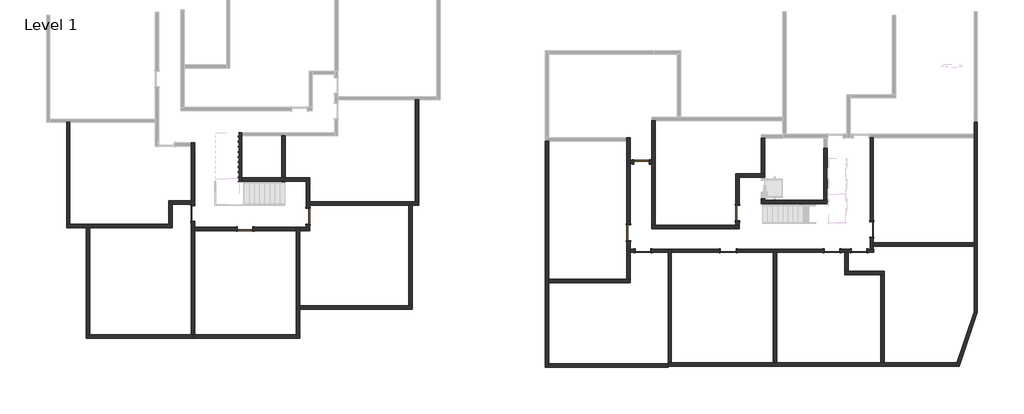
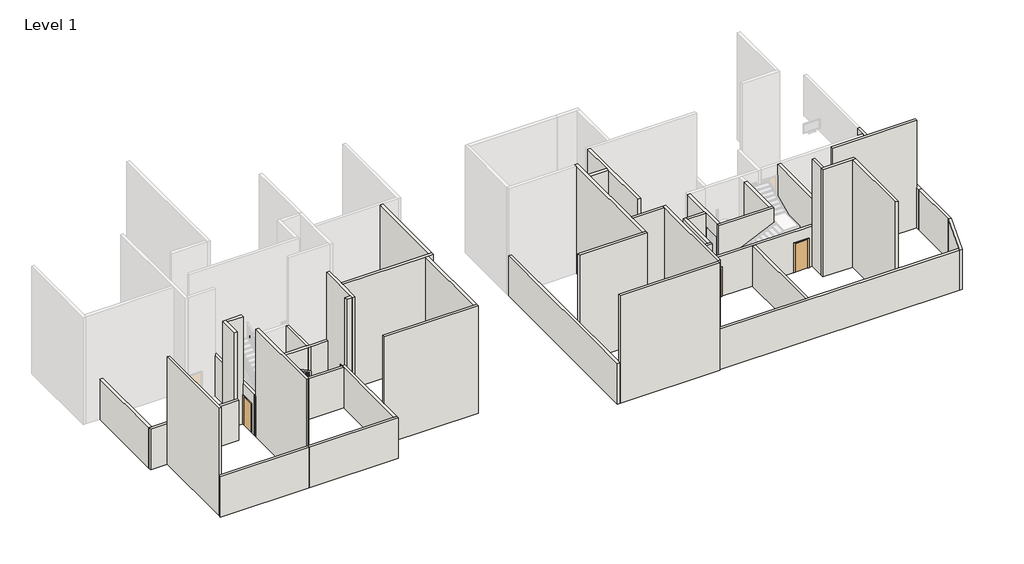
# One storey, part 1 of 3: 45 walls, 11 doors.
"""IFC4 building model written with IfcOpenShell, lengths in millimetres."""

import ifcopenshell
import ifcopenshell.guid

model = None  # the IFC model being written
_history = None  # IfcOwnerHistory: only IFC2X3 demands one
_inside = {}  # id of a spatial element -> (the spatial element, [elements in it])
_under = {}  # id of a project, library or spatial element -> (it, [spatial elements below it])
_declared = {}  # id of a project -> (the project, [libraries it declares])
_typed = {}  # id of a type object -> (the type object, [elements of that type])
_made_of = {}  # id of a material, layer set ... -> (it, [elements and type objects made of it])


def new_model(schema):
    """Start an empty IFC model of exactly this schema.

    Asked for "IFC4X3", IfcOpenShell would pick the latest addendum, in which some entities
    have other attributes; the version numbers below select the first issue.
    IFC2X3 requires an IfcOwnerHistory on every rooted entity: one is made here for all.
    """
    global model, _history
    if schema == "IFC4X3":
        model = ifcopenshell.file(schema_version=(4, 3, 0, 0))
    else:
        model = ifcopenshell.file(schema=schema)
    _inside.clear()
    _under.clear()
    _declared.clear()
    _typed.clear()
    _made_of.clear()
    _history = None
    if model.schema == "IFC2X3":
        org = make("IfcOrganization", Name="unknown")
        user = make(
            "IfcPersonAndOrganization",
            ThePerson=make("IfcPerson", FamilyName="unknown"),
            TheOrganization=org,
        )
        app = make(
            "IfcApplication",
            ApplicationDeveloper=org,
            Version="unknown",
            ApplicationFullName="unknown",
            ApplicationIdentifier="unknown",
        )
        _history = make(
            "IfcOwnerHistory",
            OwningUser=user,
            OwningApplication=app,
            ChangeAction="ADDED",
            CreationDate=0,
        )
    return model


def make(cls, **values):
    """One entity of the class cls with the attributes given. An attribute that is None is left unset."""
    return model.create_entity(
        cls, **{name: value for name, value in values.items() if value is not None}
    )


def rooted(cls, **values):
    """An entity with a GlobalId (a new one), such as an element, a storey or a relation."""
    return make(cls, GlobalId=ifcopenshell.guid.new(), OwnerHistory=_history, **values)


def si_unit(unit_type, name, prefix=None):
    """IfcSIUnit, for example si_unit("LENGTHUNIT", "METRE", prefix="MILLI")."""
    return make("IfcSIUnit", UnitType=unit_type, Prefix=prefix, Name=name)


def assignment(units):
    """IfcUnitAssignment: the units of a project."""
    return None if units is None else make("IfcUnitAssignment", Units=units)


def point(xyz):
    """IfcCartesianPoint."""
    return None if xyz is None else make("IfcCartesianPoint", Coordinates=xyz)


def direction(xyz):
    """IfcDirection."""
    return None if xyz is None else make("IfcDirection", DirectionRatios=xyz)


def frame(location, z_axis=None, x_axis=None):
    """IfcAxis2Placement3D, a coordinate frame: its origin and axes. An axis left out is left unset."""
    return make(
        "IfcAxis2Placement3D",
        Location=point(location),
        Axis=direction(z_axis),
        RefDirection=direction(x_axis),
    )


def origin():
    """The frame at (0, 0, 0) with its axes left unset."""
    return frame((0.0, 0.0, 0.0))


def origin_with_axes():
    """The frame at (0, 0, 0) with the z axis (0, 0, 1) and the x axis (1, 0, 0) written out."""
    return frame((0.0, 0.0, 0.0), z_axis=(0.0, 0.0, 1.0), x_axis=(1.0, 0.0, 0.0))


def place(relative_to, where):
    """IfcLocalPlacement: puts the frame where relative to a parent placement (None: the world)."""
    return make(
        "IfcLocalPlacement", PlacementRelTo=relative_to, RelativePlacement=where
    )


def context(
    kind, dimensions, precision=None, world=None, true_north=None, identifier=None
):
    """IfcGeometricRepresentationContext, for example the 3D "Model" context."""
    return make(
        "IfcGeometricRepresentationContext",
        ContextIdentifier=identifier,
        ContextType=kind,
        CoordinateSpaceDimension=dimensions,
        Precision=precision,
        WorldCoordinateSystem=world,
        TrueNorth=true_north,
    )


def project(units=None, contexts=None):
    """IfcProject with its units and contexts."""
    return rooted(
        "IfcProject",
        Name="project",
        RepresentationContexts=contexts,
        UnitsInContext=assignment(units),
    )


def spatial(cls, under=None, at=None, **own):
    """A site, building, storey or space (cls), placed at a placement, below another one or the project."""
    s = rooted(cls, ObjectPlacement=at, **own)
    if under is not None:
        _under.setdefault(under.id(), (under, []))[1].append(s)
    return s


def polyline(points):
    """IfcPolyline through the points."""
    return make("IfcPolyline", Points=[point(p) for p in points])


def outline(outer, holes=None, kind="AREA"):
    """IfcArbitraryClosedProfileDef: a profile drawn as a closed curve; with holes, ...WithVoids."""
    if holes is None:
        return make("IfcArbitraryClosedProfileDef", ProfileType=kind, OuterCurve=outer)
    return make(
        "IfcArbitraryProfileDefWithVoids",
        ProfileType=kind,
        OuterCurve=outer,
        InnerCurves=holes,
    )


def extrude(swept, where, along, depth):
    """IfcExtrudedAreaSolid: the profile swept, set in the frame where, extruded along a direction by depth."""
    return make(
        "IfcExtrudedAreaSolid",
        SweptArea=swept,
        Position=where,
        ExtrudedDirection=direction(along),
        Depth=depth,
    )


def faces_of(points, faces, orient=None, outer=None):
    """IfcFace entities. A face is a list of loops; a loop is a list of indices into points, from 0.

    orient and outer hold one flag for each loop. By default every Orientation is true, the
    first loop of a face is its IfcFaceOuterBound and the others are IfcFaceBound.
    """
    made = []
    for i, loops in enumerate(faces):
        bounds = []
        for j, loop in enumerate(loops):
            is_outer = j == 0 if outer is None else outer[i][j]
            bounds.append(
                make(
                    "IfcFaceOuterBound" if is_outer else "IfcFaceBound",
                    Bound=make("IfcPolyLoop", Polygon=[points[k] for k in loop]),
                    Orientation=True if orient is None else orient[i][j],
                )
            )
        made.append(make("IfcFace", Bounds=bounds))
    return made


def faceted_brep(points, faces, orient=None, outer=None, voids=None):
    """IfcFacetedBrep: a solid bounded by flat faces; with voids (closed shells), ...WithVoids."""
    shared = [point(p) for p in points]
    hull = make("IfcClosedShell", CfsFaces=faces_of(shared, faces, orient, outer))
    if voids is None:
        return make("IfcFacetedBrep", Outer=hull)
    return make(
        "IfcFacetedBrepWithVoids",
        Outer=hull,
        Voids=[
            make(cls, CfsFaces=faces_of(shared, fs, o, b)) for cls, fs, o, b in voids
        ],
    )


def shape(context_of_items, identifier, shape_type, items):
    """IfcShapeRepresentation: the items that make up one representation, for example the "Body"."""
    return make(
        "IfcShapeRepresentation",
        ContextOfItems=context_of_items,
        RepresentationIdentifier=identifier,
        RepresentationType=shape_type,
        Items=items,
    )


def source(mapping_origin, context_of_items, identifier, shape_type, items):
    """IfcRepresentationMap: a shape defined once, which mapped items show again and again."""
    return make(
        "IfcRepresentationMap",
        MappingOrigin=mapping_origin,
        MappedRepresentation=shape(context_of_items, identifier, shape_type, items),
    )


def transform(
    local_origin,
    x_axis=None,
    y_axis=None,
    z_axis=None,
    scale=None,
    scale2=None,
    scale3=None,
    uniform=True,
):
    """IfcCartesianTransformationOperator3D, or its non-uniform kind. x_axis, y_axis, z_axis: its Axis1, 2, 3."""
    if uniform:
        return make(
            "IfcCartesianTransformationOperator3D",
            Axis1=direction(x_axis),
            Axis2=direction(y_axis),
            LocalOrigin=point(local_origin),
            Scale=scale,
            Axis3=direction(z_axis),
        )
    return make(
        "IfcCartesianTransformationOperator3DnonUniform",
        Axis1=direction(x_axis),
        Axis2=direction(y_axis),
        LocalOrigin=point(local_origin),
        Scale=scale,
        Axis3=direction(z_axis),
        Scale2=scale2,
        Scale3=scale3,
    )


def mapped(mapping_source, mapping_target):
    """IfcMappedItem: shows the shape of a source again, moved by a transform."""
    return make(
        "IfcMappedItem", MappingSource=mapping_source, MappingTarget=mapping_target
    )


def made_of(thing, what):
    """Note that an element or type object is made of a material, layer set ...; save() writes the relation."""
    if what is not None:
        _made_of.setdefault(what.id(), (what, []))[1].append(thing)
    return thing


def element(
    cls,
    number,
    at=None,
    inside=None,
    cuts=None,
    type_object=None,
    material=None,
    context=None,
    identifier="Body",
    shape_type=None,
    held_by="IfcProductDefinitionShape",
    body=None,
    shapes=None,
    **own,
):
    """One element of the class cls, such as IfcWall. Its Tag is "e" and its number.

    at: its placement. inside: the storey or other place that contains it. cuts: it is an
    opening in that element (IfcRelVoidsElement). A single representation is given by context,
    identifier, shape_type and body (its items); several are given by shapes. held_by: the class
    of the entity that holds the representations. save() writes the other relations.
    """
    e = rooted(cls, Tag="e%d" % number, ObjectPlacement=at, **own)
    if body is not None:
        shapes = [shape(context, identifier, shape_type, body)]
    if shapes is not None:
        e.Representation = make(held_by, Representations=shapes)
    if inside is not None:
        _inside.setdefault(inside.id(), (inside, []))[1].append(e)
    if cuts is not None:
        rooted(
            "IfcRelVoidsElement", RelatingBuildingElement=cuts, RelatedOpeningElement=e
        )
    if type_object is not None:
        _typed.setdefault(type_object.id(), (type_object, []))[1].append(e)
    return made_of(e, material)


def aggregate(whole, parts):
    """IfcRelAggregates: a whole, such as a stair, and the parts it consists of."""
    return rooted("IfcRelAggregates", RelatingObject=whole, RelatedObjects=parts)


def save(model, path):
    """Write the relations noted so far, then the file.

    IfcRelAggregates (storeys below a building ...), IfcRelContainedInSpatialStructure (elements
    in a storey), IfcRelDefinesByType, IfcRelAssociatesMaterial and IfcRelDeclares: one each for
    every whole, place, type object, material and project.
    """
    for whole, parts in _under.values():
        aggregate(whole, parts)
    for where, things in _inside.values():
        rooted(
            "IfcRelContainedInSpatialStructure",
            RelatedElements=things,
            RelatingStructure=where,
        )
    for kind, things in _typed.values():
        rooted("IfcRelDefinesByType", RelatedObjects=things, RelatingType=kind)
    for what, things in _made_of.values():
        rooted("IfcRelAssociatesMaterial", RelatedObjects=things, RelatingMaterial=what)
    for by, libraries in _declared.values():
        rooted("IfcRelDeclares", RelatingContext=by, RelatedDefinitions=libraries)
    model.write(path)


def m_single_flush_0915_x_2134mm_727434cd(model_context):
    return source(origin(), model_context, "Body", "SweptSolid", [
        extrude(outline(polyline([(2210.0, -533.5), (0.0, -533.5), (0.0, -457.5), (2134.0, -457.5), (2134.0, 457.5), (0.0, 457.5), (0.0, 533.5), (2210.0, 533.5), (2210.0, -533.5)])), frame((0.0, -125.0, 0.0), z_axis=(0.0, 1.0, 0.0), x_axis=(0.0, 0.0, 1.0)), (0.0, 0.0, 1.0), 25.0),
        extrude(outline(polyline([(2210.0, 533.5), (2210.0, -533.5), (0.0, -533.5), (0.0, -457.5), (2134.0, -457.5), (2134.0, 457.5), (0.0, 457.5), (0.0, 533.5), (2210.0, 533.5)])), frame((0.0, 100.0, 0.0), z_axis=(0.0, 1.0, 0.0), x_axis=(0.0, 0.0, 1.0)), (0.0, 0.0, 1.0), 25.0),
        extrude(outline(polyline([(457.5, -49.0), (457.5, -100.0), (-457.5, -100.0), (-457.5, -49.0), (457.5, -49.0)])), origin_with_axes(), (0.0, 0.0, 1.0), 2134.0),
    ])


def m_single_flush_0915_x_2134mm_6a9e8738(model_context):
    return source(origin(), model_context, "Body", "SweptSolid", [
        extrude(outline(polyline([(2210.0, -533.5), (0.0, -533.5), (0.0, -457.5), (2134.0, -457.5), (2134.0, 457.5), (0.0, 457.5), (0.0, 533.5), (2210.0, 533.5), (2210.0, -533.5)])), frame((0.0, 100.0, 0.0), z_axis=(0.0, 1.0, 0.0), x_axis=(0.0, 0.0, 1.0)), (0.0, 0.0, 1.0), 25.0),
        extrude(outline(polyline([(2210.0, 533.5), (2210.0, -533.5), (0.0, -533.5), (0.0, -457.5), (2134.0, -457.5), (2134.0, 457.5), (0.0, 457.5), (0.0, 533.5), (2210.0, 533.5)])), frame((0.0, -125.0, 0.0), z_axis=(0.0, 1.0, 0.0), x_axis=(0.0, 0.0, 1.0)), (0.0, 0.0, 1.0), 25.0),
        extrude(outline(polyline([(457.5, 49.0), (-457.5, 49.0), (-457.5, 100.0), (457.5, 100.0), (457.5, 49.0)])), origin_with_axes(), (0.0, 0.0, 1.0), 2134.0),
    ])


model = new_model("IFC4")

# Units and contexts
model_context = context("Model", 3, world=origin())
ifc_project = project(units=[si_unit("LENGTHUNIT", "METRE", prefix="MILLI")], contexts=[model_context])

# Site, building, storey
site = spatial("IfcSite", under=ifc_project)
building = spatial("IfcBuilding", under=site)
storey = spatial("IfcBuildingStorey", under=building, Name="Level 1", Elevation=0.0)

# Doors
placement = place(None, origin())
m_single_flush_0915_x_2134mm_shape = m_single_flush_0915_x_2134mm_727434cd(model_context)
element("IfcDoor", 1, ObjectType="M_Single-Flush : 0915 x 2134mm", at=placement, inside=storey, context=model_context, shape_type="MappedRepresentation", body=[
    mapped(m_single_flush_0915_x_2134mm_shape, transform((16150.6041014, -4023.024372, 0.0), x_axis=(0.0, -1.0, 0.0), y_axis=(1.0, 0.0, 0.0), z_axis=(0.0, 0.0, 1.0))),
])
element("IfcDoor", 2, ObjectType="M_Single-Flush : 0915 x 2134mm", at=placement, inside=storey, context=model_context, shape_type="MappedRepresentation", body=[
    mapped(m_single_flush_0915_x_2134mm_shape, transform((15602.336337, -6240.0098119, 0.0), x_axis=(1.0, 0.0, 0.0), y_axis=(0.0, 1.0, 0.0), z_axis=(0.0, 0.0, 1.0))),
])
element("IfcDoor", 3, ObjectType="M_Single-Flush : 0915 x 2134mm", at=placement, inside=storey, context=model_context, shape_type="MappedRepresentation", body=[
    mapped(m_single_flush_0915_x_2134mm_shape, transform((21711.3612349, -6240.0098119, 0.0), x_axis=(1.0, 0.0, 0.0), y_axis=(0.0, 1.0, 0.0), z_axis=(0.0, 0.0, 1.0))),
])
element("IfcDoor", 4, ObjectType="M_Single-Flush : 0915 x 2134mm", at=placement, inside=storey, context=model_context, shape_type="MappedRepresentation", body=[
    mapped(m_single_flush_0915_x_2134mm_shape, transform((-9130.3629108, -4209.1627129, 0.0), x_axis=(0.0, 1.0, 0.0), y_axis=(-1.0, 0.0, 0.0), z_axis=(0.0, 0.0, 1.0))),
])
m_single_flush_0915_x_2134mm_2_shape = m_single_flush_0915_x_2134mm_6a9e8738(model_context)
element("IfcDoor", 5, ObjectType="M_Single-Flush : 0915 x 2134mm", at=placement, inside=storey, context=model_context, shape_type="MappedRepresentation", body=[
    mapped(m_single_flush_0915_x_2134mm_2_shape, transform((24048.8612349, -4982.5098119, 0.0), x_axis=(0.0, -1.0, 0.0), y_axis=(1.0, 0.0, 0.0), z_axis=(0.0, 0.0, 1.0))),
])
element("IfcDoor", 6, ObjectType="M_Single-Flush : 0915 x 2134mm", at=placement, inside=storey, context=model_context, shape_type="MappedRepresentation", body=[
    mapped(m_single_flush_0915_x_2134mm_2_shape, transform((23308.8612349, -6240.0098119, 0.0), x_axis=(-1.0, 0.0, 0.0), y_axis=(0.0, -1.0, 0.0), z_axis=(0.0, 0.0, 1.0))),
])
element("IfcDoor", 7, ObjectType="M_Single-Flush : 0915 x 2134mm", at=placement, inside=storey, context=model_context, shape_type="MappedRepresentation", body=[
    mapped(m_single_flush_0915_x_2134mm_2_shape, transform((-12832.3304233, -4959.1627129, 0.0), x_axis=(-1.0, 0.0, 0.0), y_axis=(0.0, -1.0, 0.0), z_axis=(0.0, 0.0, 1.0))),
])
element("IfcDoor", 8, ObjectType="M_Single-Flush : 0915 x 2134mm", at=placement, inside=storey, context=model_context, shape_type="MappedRepresentation", body=[
    mapped(m_single_flush_0915_x_2134mm_2_shape, transform((10586.3612349, -6236.6907835, 0.0), x_axis=(-1.0, 0.0, 0.0), y_axis=(0.0, -1.0, 0.0), z_axis=(0.0, 0.0, 1.0))),
])
element("IfcDoor", 9, ObjectType="M_Single-Flush : 0915 x 2134mm", at=placement, inside=storey, context=model_context, shape_type="MappedRepresentation", body=[
    mapped(m_single_flush_0915_x_2134mm_2_shape, transform((9728.8612349, -5179.1907835, 0.0), x_axis=(0.0, 1.0, 0.0), y_axis=(-1.0, 0.0, 0.0), z_axis=(0.0, 0.0, 1.0))),
])
element("IfcDoor", 10, ObjectType="M_Single-Flush : 0915 x 2134mm", at=placement, inside=storey, context=model_context, shape_type="MappedRepresentation", body=[
    mapped(m_single_flush_0915_x_2134mm_2_shape, transform((10497.5506524, -1020.524372, 0.0), x_axis=(1.0, 0.0, 0.0), y_axis=(0.0, 1.0, 0.0), z_axis=(0.0, 0.0, 1.0))),
])
element("IfcDoor", 11, ObjectType="M_Single-Flush : 0915 x 2134mm", at=placement, inside=storey, context=model_context, shape_type="MappedRepresentation", body=[
    mapped(m_single_flush_0915_x_2134mm_2_shape, transform((-15913.9741722, -4044.6599715, 0.0), x_axis=(0.0, 1.0, 0.0), y_axis=(-1.0, 0.0, 0.0), z_axis=(0.0, 0.0, 1.0))),
])

# Walls
element("IfcWall", 12, ObjectType="Generic - 200mm", at=placement, inside=storey, context=model_context, shape_type="Brep", body=[
    faceted_brep([(30068.8612349, 1319.475628, 0.0), (30068.8612349, 619.475628, 0.0), (30068.8612349, 419.475628, 0.0), (30068.8612349, -5760.0098119, 0.0), (30068.8612349, -5960.0098119, 0.0), (30068.8612349, -6240.0098119, 0.0), (30068.8612349, -6240.0098119, 3000.0), (30068.8612349, 419.475628, 3000.0), (30068.8612349, 619.475628, 3000.0), (30068.8612349, 1319.475628, 3000.0), (30268.8612349, 1319.475628, 0.0), (30268.8612349, 1319.475628, 3000.0), (30268.8612349, -6240.0098119, 3000.0), (30268.8612349, -6240.0098119, 0.0), (30268.3425199, 1319.475628, 0.0), (30069.3799498, -6240.0098119, 0.0), (30069.3799498, -6240.0098119, 3000.0), (30268.3425199, 1319.475628, 3000.0)], [[[0, 1, 2, 3, 4, 5, 6, 7, 8, 9]], [[10, 11, 12, 13]], [[5, 4, 3, 2, 1, 0, 14, 10, 13, 15]], [[6, 5, 15, 13, 12, 16]], [[9, 8, 7, 6, 16, 12, 11, 17]], [[0, 9, 17, 11, 10, 14]]]),
])
element("IfcWall", 13, ObjectType="Generic - 200mm", at=placement, inside=storey, context=model_context, shape_type="Brep", body=[
    faceted_brep([(30069.3799498, -6240.0098119, 0.0), (30069.3799498, -9831.8731192, 0.0), (30069.3799498, -9831.8731192, 3000.0), (30069.3799498, -6240.0098119, 3000.0), (30269.3799498, -6240.0098119, 0.0), (30269.3799498, -6240.0098119, 3000.0), (30269.3799498, -9864.7113693, 3000.0), (30269.3799498, -9864.7113693, 0.0), (30268.8612349, -6240.0098119, 0.0), (30268.8612349, -6240.0098119, 3000.0)], [[[0, 1, 2, 3]], [[4, 5, 6, 7]], [[1, 0, 8, 4, 7]], [[3, 2, 6, 5, 9]], [[0, 3, 9, 5, 4, 8]], [[2, 1, 7, 6]]]),
])
element("IfcWall", 14, ObjectType="Generic - 200mm", at=placement, inside=storey, context=model_context, shape_type="Brep", body=[
    faceted_brep([(21429.836337, -3276.2808257, 0.0), (21229.836337, -3276.2808257, 0.0), (17750.6041014, -3276.2808257, 0.0), (17550.6041014, -3276.2808257, 0.0), (17550.6041014, -3276.2808257, 3000.0), (17750.6041014, -3276.2808257, 3000.0), (21229.836337, -3276.2808257, 3000.0), (21429.836337, -3276.2808257, 3000.0), (21429.836337, -3476.2808257, 0.0), (21429.836337, -3476.2808257, 3000.0), (17550.6041014, -3476.2808257, 3000.0), (17550.6041014, -3476.2808257, 0.0)], [[[0, 1, 2, 3, 4, 5, 6, 7]], [[8, 9, 10, 11]], [[3, 2, 1, 0, 8, 11]], [[7, 6, 5, 4, 10, 9]], [[0, 7, 9, 8]], [[4, 3, 11, 10]]]),
])
element("IfcWall", 15, ObjectType="Generic - 200mm", at=placement, inside=storey, context=model_context, shape_type="SweptSolid", body=[
    extrude(outline(polyline([(18459.836337, -6340.0098119), (18459.836337, -12836.6907835), (18259.836337, -12836.6907835), (18259.836337, -6340.0098119), (18459.836337, -6340.0098119)])), origin_with_axes(), (0.0, 0.0, 1.0), 3000.0),
])
element("IfcWall", 16, ObjectType="Generic - 200mm", at=placement, inside=storey, context=model_context, shape_type="Brep", body=[
    faceted_brep([(29055.3124022, -12836.6907835, 0.0), (24788.8612349, -12836.6907835, 0.0), (24588.8612349, -12836.6907835, 0.0), (18459.836337, -12836.6907835, 0.0), (18259.836337, -12836.6907835, 0.0), (12259.836337, -12836.6907835, 0.0), (12059.836337, -12836.6907835, 0.0), (12059.836337, -12836.6907835, 3000.0), (18259.836337, -12836.6907835, 3000.0), (18459.836337, -12836.6907835, 3000.0), (29055.3124022, -12836.6907835, 3000.0), (28987.8162902, -13036.6907835, 0.0), (28987.8162902, -13036.6907835, 3000.0), (12059.836337, -13036.6907835, 3000.0), (12059.836337, -13036.6907835, 0.0), (12059.836337, -12889.1627129, 0.0)], [[[0, 1, 2, 3, 4, 5, 6, 7, 8, 9, 10]], [[11, 12, 13, 14]], [[6, 5, 4, 3, 2, 1, 0, 11, 14, 15]], [[10, 9, 8, 7, 13, 12]], [[0, 10, 12, 11]], [[7, 6, 15, 14, 13]]]),
])
element("IfcWall", 17, ObjectType="Generic - 200mm", at=placement, inside=storey, context=model_context, shape_type="Brep", body=[
    faceted_brep([(30069.3799498, -9831.8731192, 0.0), (29055.3124022, -12836.6907835, 0.0), (28987.8162902, -13036.6907835, 0.0), (28987.8162902, -13036.6907835, 3000.0), (29055.3124022, -12836.6907835, 3000.0), (30069.3799498, -9831.8731192, 3000.0), (30269.3799498, -9864.7113693, 0.0), (30269.3799498, -9864.7113693, 3000.0), (29198.8985612, -13036.6907835, 3000.0), (29198.8985612, -13036.6907835, 0.0)], [[[0, 1, 2, 3, 4, 5]], [[6, 7, 8, 9]], [[2, 1, 0, 6, 9]], [[5, 4, 3, 8, 7]], [[0, 5, 7, 6]], [[3, 2, 9, 8]]]),
])
element("IfcWall", 18, ObjectType="Generic - 200mm", at=placement, inside=storey, context=model_context, shape_type="Brep", body=[
    faceted_brep([(22851.3612349, -6140.0098119, 0.0), (22168.8612349, -6140.0098119, 0.0), (22168.8612349, -6140.0098119, 2134.0), (21253.8612349, -6140.0098119, 2134.0), (21253.8612349, -6140.0098119, 0.0), (16059.836337, -6140.0098119, 0.0), (16059.836337, -6140.0098119, 2134.0), (15144.836337, -6140.0098119, 2134.0), (15144.836337, -6140.0098119, 0.0), (12259.836337, -6140.0098119, 0.0), (12259.836337, -6140.0098119, 3000.0), (23948.8612349, -6140.0098119, 3000.0), (24148.8612349, -6140.0098119, 3000.0), (24163.3998354, -6140.0098119, 3000.0), (24163.3998354, -6140.0098119, 0.0), (24148.8612349, -6140.0098119, 0.0), (23948.8612349, -6140.0098119, 0.0), (23766.3612349, -6140.0098119, 0.0), (23766.3612349, -6140.0098119, 2134.0), (22851.3612349, -6140.0098119, 2134.0), (22168.8612349, -6340.0098119, 2134.0), (22168.8612349, -6340.0098119, 0.0), (22468.8612349, -6340.0098119, 0.0), (22668.8612349, -6340.0098119, 0.0), (22851.3612349, -6340.0098119, 0.0), (22851.3612349, -6340.0098119, 2134.0), (23766.3612349, -6340.0098119, 2134.0), (23766.3612349, -6340.0098119, 0.0), (24163.3998354, -6340.0098119, 0.0), (24163.3998354, -6340.0098119, 3000.0), (18459.836337, -6340.0098119, 3000.0), (18259.836337, -6340.0098119, 3000.0), (12259.836337, -6340.0098119, 3000.0), (12259.836337, -6340.0098119, 0.0), (15144.836337, -6340.0098119, 0.0), (15144.836337, -6340.0098119, 2134.0), (16059.836337, -6340.0098119, 2134.0), (16059.836337, -6340.0098119, 0.0), (18259.836337, -6340.0098119, 0.0), (18459.836337, -6340.0098119, 0.0), (21253.8612349, -6340.0098119, 0.0), (21253.8612349, -6340.0098119, 2134.0)], [[[0, 1, 2, 3, 4, 5, 6, 7, 8, 9, 10, 11, 12, 13, 14, 15, 16, 17, 18, 19]], [[20, 21, 22, 23, 24, 25, 26, 27, 28, 29, 30, 31, 32, 33, 34, 35, 36, 37, 38, 39, 40, 41]], [[17, 16, 15, 14, 28, 27]], [[33, 9, 8, 34]], [[40, 39, 38, 37, 5, 4]], [[24, 23, 22, 21, 1, 0]], [[13, 12, 11, 10, 32, 31, 30, 29]], [[14, 13, 29, 28]], [[36, 6, 5, 37]], [[7, 35, 34, 8]], [[35, 7, 6, 36]], [[25, 24, 0, 19]], [[26, 25, 19, 18]], [[27, 26, 18, 17]], [[10, 9, 33, 32]], [[2, 1, 21, 20]], [[3, 2, 20, 41]], [[4, 3, 41, 40]]]),
])
element("IfcWall", 19, ObjectType="Generic - 200mm", at=placement, inside=storey, context=model_context, shape_type="Brep", body=[
    faceted_brep([(4843.716007, 199.9901881, 0.0), (4843.716007, -13089.1627129, 0.0), (4843.716007, -13089.1627129, 3000.0), (4843.716007, 199.9901881, 3000.0), (5043.716007, 199.9901881, 0.0), (5043.716007, 199.9901881, 3000.0), (5043.716007, -13089.1627129, 3000.0), (5043.716007, -13089.1627129, 0.0), (5043.716007, -12889.1627129, 0.0), (5043.716007, -8120.0098119, 0.0), (5043.716007, -7920.0098119, 0.0)], [[[0, 1, 2, 3]], [[4, 5, 6, 7, 8, 9, 10]], [[1, 0, 4, 10, 9, 8, 7]], [[3, 2, 6, 5]], [[0, 3, 5, 4]], [[2, 1, 7, 6]]]),
])
element("IfcWall", 20, ObjectType="Generic - 200mm", at=placement, inside=storey, context=model_context, shape_type="Brep", body=[
    faceted_brep([(24148.8612349, 419.475628, 3000.0), (24148.8612349, -6140.0098119, 3000.0), (24148.8612349, -6140.0098119, 0.0), (24148.8612349, -5960.0098119, 0.0), (24148.8612349, -5760.0098119, 0.0), (24148.8612349, -5440.0098119, 0.0), (24148.8612349, -5440.0098119, 2134.0), (24148.8612349, -4525.0098119, 2134.0), (24148.8612349, -4525.0098119, 0.0), (24148.8612349, 419.475628, 0.0), (23948.8612349, -6140.0098119, 3000.0), (23948.8612349, 419.475628, 3000.0), (23948.8612349, 419.475628, 0.0), (23948.8612349, -4525.0098119, 0.0), (23948.8612349, -4525.0098119, 2134.0), (23948.8612349, -5440.0098119, 2134.0), (23948.8612349, -5440.0098119, 0.0), (23948.8612349, -6140.0098119, 0.0)], [[[0, 1, 2, 3, 4, 5, 6, 7, 8, 9]], [[10, 11, 12, 13, 14, 15, 16, 17]], [[12, 9, 8, 13]], [[2, 17, 16, 5, 4, 3]], [[1, 0, 11, 10]], [[0, 9, 12, 11]], [[15, 6, 5, 16]], [[7, 14, 13, 8]], [[14, 7, 6, 15]], [[2, 1, 10, 17]]]),
])
element("IfcWall", 21, ObjectType="Generic - 200mm", at=placement, inside=storey, context=model_context, shape_type="SweptSolid", body=[
    extrude(outline(polyline([(21229.836337, -3276.2808257), (21229.836337, -200.524372), (21429.836337, -200.524372), (21429.836337, -3276.2808257), (21229.836337, -3276.2808257)])), origin_with_axes(), (0.0, 0.0, 1.0), 3000.0),
])
element("IfcWall", 22, ObjectType="Generic - 200mm", at=placement, inside=storey, context=model_context, shape_type="Brep", body=[
    faceted_brep([(17550.6041014, -3276.2808257, 3000.0), (17550.6041014, -1920.524372, 3000.0), (17550.6041014, -1720.524372, 3000.0), (17550.6041014, 379.475628, 3000.0), (17550.6041014, 379.475628, 0.0), (17550.6041014, -1720.524372, 0.0), (17550.6041014, -1920.524372, 0.0), (17550.6041014, -1926.2808257, 0.0), (17550.6041014, -1926.2808257, 2000.0), (17550.6041014, -3181.2876228, 2000.0), (17550.6041014, -3181.2876228, 0.0), (17550.6041014, -3276.2808257, 0.0), (17750.6041014, 379.475628, 3000.0), (17750.6041014, -3276.2808257, 3000.0), (17750.6041014, -3276.2808257, 0.0), (17750.6041014, -3181.2876228, 0.0), (17750.6041014, -3181.2876228, 2000.0), (17750.6041014, -1926.2808257, 2000.0), (17750.6041014, -1926.2808257, 0.0), (17750.6041014, 379.475628, 0.0)], [[[0, 1, 2, 3, 4, 5, 6, 7, 8, 9, 10, 11]], [[12, 13, 14, 15, 16, 17, 18, 19]], [[14, 11, 10, 15]], [[4, 19, 18, 7, 6, 5]], [[3, 2, 1, 0, 13, 12]], [[0, 11, 14, 13]], [[9, 16, 15, 10]], [[17, 8, 7, 18]], [[8, 17, 16, 9]], [[4, 3, 12, 19]]]),
])
element("IfcWall", 23, ObjectType="Generic - 200mm", at=placement, inside=storey, context=model_context, shape_type="Brep", body=[
    faceted_brep([(11108.8612349, -4940.0098119, 0.0), (16250.6041014, -4940.0098119, 0.0), (16250.6041014, -4940.0098119, 3000.0), (11108.8612349, -4940.0098119, 3000.0), (11108.8612349, -4740.0098119, 0.0), (11108.8612349, -4740.0098119, 3000.0), (16050.6041014, -4740.0098119, 3000.0), (16250.6041014, -4740.0098119, 3000.0), (16250.6041014, -4740.0098119, 0.0), (16050.6041014, -4740.0098119, 0.0), (11308.8612349, -4740.0098119, 0.0)], [[[0, 1, 2, 3]], [[4, 5, 6, 7, 8, 9, 10]], [[1, 0, 4, 10, 9, 8]], [[3, 2, 7, 6, 5]], [[2, 1, 8, 7]], [[0, 3, 5, 4]]]),
])
element("IfcWall", 24, ObjectType="Generic - 200mm", at=placement, inside=storey, context=model_context, shape_type="Brep", body=[
    faceted_brep([(16250.6041014, -1720.524372, 3000.0), (16250.6041014, -1920.524372, 3000.0), (16250.6041014, -4740.0098119, 3000.0), (16250.6041014, -4740.0098119, 0.0), (16250.6041014, -4480.524372, 0.0), (16250.6041014, -4480.524372, 2134.0), (16250.6041014, -3565.524372, 2134.0), (16250.6041014, -3565.524372, 0.0), (16250.6041014, -1920.524372, 0.0), (16250.6041014, -1720.524372, 0.0), (16050.6041014, -4740.0098119, 3000.0), (16050.6041014, -1720.524372, 3000.0), (16050.6041014, -1720.524372, 0.0), (16050.6041014, -3565.524372, 0.0), (16050.6041014, -3565.524372, 2134.0), (16050.6041014, -4480.524372, 2134.0), (16050.6041014, -4480.524372, 0.0), (16050.6041014, -4740.0098119, 0.0)], [[[0, 1, 2, 3, 4, 5, 6, 7, 8, 9]], [[10, 11, 12, 13, 14, 15, 16, 17]], [[3, 17, 16, 4]], [[12, 9, 8, 7, 13]], [[2, 1, 0, 11, 10]], [[3, 2, 10, 17]], [[0, 9, 12, 11]], [[15, 5, 4, 16]], [[6, 14, 13, 7]], [[14, 6, 5, 15]]]),
])
element("IfcWall", 25, ObjectType="Generic - 200mm", at=placement, inside=storey, context=model_context, shape_type="SweptSolid", body=[
    extrude(outline(polyline([(17550.6041014, -1920.524372), (16250.6041014, -1920.524372), (16250.6041014, -1720.524372), (17550.6041014, -1720.524372), (17550.6041014, -1920.524372)])), origin_with_axes(), (0.0, 0.0, 1.0), 3000.0),
])
element("IfcWall", 26, ObjectType="Generic - 200mm", at=placement, inside=storey, context=model_context, shape_type="Brep", body=[
    faceted_brep([(22468.8612349, -7641.2808257, 0.0), (24588.8612349, -7641.2808257, 0.0), (24788.8612349, -7641.2808257, 0.0), (24788.8612349, -7641.2808257, 8000.0), (24588.8612349, -7641.2808257, 8000.0), (22468.8612349, -7641.2808257, 8000.0), (22468.8612349, -7441.2808257, 0.0), (22468.8612349, -7441.2808257, 8000.0), (22668.8612349, -7441.2808257, 8000.0), (24788.8612349, -7441.2808257, 8000.0), (24788.8612349, -7441.2808257, 0.0), (22668.8612349, -7441.2808257, 0.0)], [[[0, 1, 2, 3, 4, 5]], [[6, 7, 8, 9, 10, 11]], [[2, 1, 0, 6, 11, 10]], [[5, 4, 3, 9, 8, 7]], [[3, 2, 10, 9]], [[0, 5, 7, 6]]]),
])
element("IfcWall", 27, ObjectType="Generic - 200mm", at=placement, inside=storey, context=model_context, shape_type="SweptSolid", body=[
    extrude(outline(polyline([(24588.8612349, -12836.6907835), (24588.8612349, -7641.2808257), (24788.8612349, -7641.2808257), (24788.8612349, -12836.6907835), (24588.8612349, -12836.6907835)])), origin_with_axes(), (0.0, 0.0, 1.0), 8000.0),
])
element("IfcWall", 28, ObjectType="Generic - 200mm", at=placement, inside=storey, context=model_context, shape_type="SweptSolid", body=[
    extrude(outline(polyline([(22668.8612349, -6340.0098119), (22668.8612349, -7441.2808257), (22468.8612349, -7441.2808257), (22468.8612349, -6340.0098119), (22668.8612349, -6340.0098119)])), origin_with_axes(), (0.0, 0.0, 1.0), 8000.0),
])
element("IfcWall", 29, ObjectType="Generic - 200mm", at=placement, inside=storey, context=model_context, shape_type="SweptSolid", body=[
    extrude(outline(polyline([(30068.8612349, -5960.0098119), (24148.8612349, -5960.0098119), (24148.8612349, -5760.0098119), (30068.8612349, -5760.0098119), (30068.8612349, -5960.0098119)])), origin_with_axes(), (0.0, 0.0, 1.0), 8000.0),
])
element("IfcWall", 30, ObjectType="Generic - 200mm", at=placement, inside=storey, context=model_context, shape_type="Brep", body=[
    faceted_brep([(9628.8612349, 399.9901881, 0.0), (9628.8612349, 199.9901881, 0.0), (9628.8612349, -4721.6907835, 0.0), (9628.8612349, -4721.6907835, 2134.0), (9628.8612349, -5636.6907835, 2134.0), (9628.8612349, -5636.6907835, 0.0), (9628.8612349, -7920.0098119, 0.0), (9628.8612349, -7920.0098119, 8000.0), (9628.8612349, 199.9901881, 8000.0), (9628.8612349, 399.9901881, 8000.0), (9828.8612349, -4721.6907835, 2134.0), (9828.8612349, -4721.6907835, 0.0), (9828.8612349, -1120.524372, 0.0), (9828.8612349, -920.524372, 0.0), (9828.8612349, 399.9901881, 0.0), (9828.8612349, 399.9901881, 8000.0), (9828.8612349, -920.524372, 8000.0), (9828.8612349, -1120.524372, 8000.0), (9828.8612349, -6136.6907835, 8000.0), (9828.8612349, -6336.6907835, 8000.0), (9828.8612349, -7920.0098119, 8000.0), (9828.8612349, -7920.0098119, 0.0), (9828.8612349, -6336.6907835, 0.0), (9828.8612349, -6136.6907835, 0.0), (9828.8612349, -5636.6907835, 0.0), (9828.8612349, -5636.6907835, 2134.0)], [[[0, 1, 2, 3, 4, 5, 6, 7, 8, 9]], [[10, 11, 12, 13, 14, 15, 16, 17, 18, 19, 20, 21, 22, 23, 24, 25]], [[14, 13, 12, 11, 2, 1, 0]], [[24, 23, 22, 21, 6, 5]], [[9, 8, 7, 20, 19, 18, 17, 16, 15]], [[0, 9, 15, 14]], [[7, 6, 21, 20]], [[3, 2, 11, 10]], [[4, 3, 10, 25]], [[5, 4, 25, 24]]]),
])
element("IfcWall", 31, ObjectType="Generic - 200mm", at=placement, inside=storey, context=model_context, shape_type="Brep", body=[
    faceted_brep([(9828.8612349, -7920.0098119, 0.0), (9628.8612349, -7920.0098119, 0.0), (5043.716007, -7920.0098119, 0.0), (5043.716007, -7920.0098119, 8000.0), (9628.8612349, -7920.0098119, 8000.0), (9828.8612349, -7920.0098119, 8000.0), (9828.8612349, -8120.0098119, 0.0), (9828.8612349, -8120.0098119, 8000.0), (5043.716007, -8120.0098119, 8000.0), (5043.716007, -8120.0098119, 0.0)], [[[0, 1, 2, 3, 4, 5]], [[6, 7, 8, 9]], [[2, 1, 0, 6, 9]], [[5, 4, 3, 8, 7]], [[3, 2, 9, 8]], [[0, 5, 7, 6]]]),
])
element("IfcWall", 32, ObjectType="Generic - 200mm", at=placement, inside=storey, context=model_context, shape_type="Brep", body=[
    faceted_brep([(-9619.8304233, -11189.1627129, 0.0), (-9819.8304233, -11189.1627129, 0.0), (-15814.8304233, -11189.1627129, 0.0), (-15914.8304233, -11189.1627129, 0.0), (-15914.8304233, -11189.1627129, 3000.0), (-9819.8304233, -11189.1627129, 3000.0), (-9619.8304233, -11189.1627129, 3000.0), (-9619.8304233, -11389.1627129, 0.0), (-9619.8304233, -11389.1627129, 3000.0), (-15914.8304233, -11389.1627129, 3000.0), (-15914.8304233, -11389.1627129, 0.0), (-15914.8304233, -11189.6814279, 0.0), (-15914.8304233, -11189.6814279, 3000.0)], [[[0, 1, 2, 3, 4, 5, 6]], [[7, 8, 9, 10]], [[3, 2, 1, 0, 7, 10, 11]], [[4, 3, 11, 10, 9, 12]], [[6, 5, 4, 12, 9, 8]], [[0, 6, 8, 7]]]),
])
element("IfcWall", 33, ObjectType="Generic - 200mm", at=placement, inside=storey, context=model_context, shape_type="Brep", body=[
    faceted_brep([(-15914.8304233, -11189.6814279, 0.0), (-16014.8304233, -11189.6814279, 0.0), (-21985.6447259, -11189.6814279, 0.0), (-22185.6447259, -11189.6814279, 0.0), (-22185.6447259, -11189.6814279, 3000.0), (-15914.8304233, -11189.6814279, 3000.0), (-15914.8304233, -11389.6814279, 0.0), (-15914.8304233, -11389.6814279, 3000.0), (-22185.6447259, -11389.6814279, 3000.0), (-22185.6447259, -11389.6814279, 0.0), (-15914.8304233, -11389.1627129, 0.0), (-15914.8304233, -11389.1627129, 3000.0)], [[[0, 1, 2, 3, 4, 5]], [[6, 7, 8, 9]], [[3, 2, 1, 0, 10, 6, 9]], [[5, 4, 8, 7, 11]], [[0, 5, 11, 7, 6, 10]], [[4, 3, 9, 8]]]),
])
element("IfcWall", 34, ObjectType="Generic - 200mm", at=placement, inside=storey, context=model_context, shape_type="Brep", body=[
    faceted_brep([(-13026.101437, -2140.1378151, 0.0), (-13026.101437, -1940.1378151, 0.0), (-13026.101437, 520.8372871, 0.0), (-13026.101437, 720.8372871, 0.0), (-13026.101437, 720.8372871, 3000.0), (-13026.101437, 520.8372871, 3000.0), (-13026.101437, -1940.1378151, 3000.0), (-13026.101437, -2140.1378151, 3000.0), (-13226.101437, -2140.1378151, 0.0), (-13226.101437, -2140.1378151, 3000.0), (-13226.101437, 720.8372871, 3000.0), (-13226.101437, 720.8372871, 0.0)], [[[0, 1, 2, 3, 4, 5, 6, 7]], [[8, 9, 10, 11]], [[3, 2, 1, 0, 8, 11]], [[7, 6, 5, 4, 10, 9]], [[0, 7, 9, 8]], [[4, 3, 11, 10]]]),
])
element("IfcWall", 35, ObjectType="Generic - 200mm", at=placement, inside=storey, context=model_context, shape_type="Brep", body=[
    faceted_brep([(-23346.5113948, -4887.1599715, 0.0), (-22185.6447259, -4887.1599715, 0.0), (-21985.6447259, -4887.1599715, 0.0), (-17123.9741722, -4887.1599715, 0.0), (-17123.9741722, -4887.1599715, 3000.0), (-23346.5113948, -4887.1599715, 3000.0), (-23346.5113948, -4687.1599715, 0.0), (-23346.5113948, -4687.1599715, 3000.0), (-23146.5113948, -4687.1599715, 3000.0), (-17123.9741722, -4687.1599715, 3000.0), (-17123.9741722, -4687.1599715, 0.0), (-17323.9741722, -4687.1599715, 0.0), (-23146.5113948, -4687.1599715, 0.0)], [[[0, 1, 2, 3, 4, 5]], [[6, 7, 8, 9, 10, 11, 12]], [[3, 2, 1, 0, 6, 12, 11, 10]], [[5, 4, 9, 8, 7]], [[0, 5, 7, 6]], [[4, 3, 10, 9]]]),
])
element("IfcWall", 36, ObjectType="Generic - 200mm", at=placement, inside=storey, context=model_context, shape_type="SweptSolid", body=[
    extrude(outline(polyline([(-23146.5113948, 1312.8400285), (-23146.5113948, -4687.1599715), (-23346.5113948, -4687.1599715), (-23346.5113948, 1312.8400285), (-23146.5113948, 1312.8400285)])), origin_with_axes(), (0.0, 0.0, 1.0), 3000.0),
])
element("IfcWall", 37, ObjectType="Generic - 200mm", at=placement, inside=storey, context=model_context, shape_type="Brep", body=[
    faceted_brep([(-15813.9741722, -3587.1599715, 2134.0), (-15813.9741722, -3587.1599715, 0.0), (-15813.9741722, 112.8400285, 0.0), (-15813.9741722, 112.8400285, 3000.0), (-15813.9741722, -4859.1627129, 3000.0), (-15813.9741722, -4859.1627129, 0.0), (-15813.9741722, -4502.1599715, 0.0), (-15813.9741722, -4502.1599715, 2134.0), (-16013.9741722, 112.8400285, 0.0), (-16013.9741722, -87.1599715, 0.0), (-16013.9741722, -3287.1599715, 0.0), (-16013.9741722, -3487.1599715, 0.0), (-16013.9741722, -3587.1599715, 0.0), (-16013.9741722, -3587.1599715, 2134.0), (-16013.9741722, -4502.1599715, 2134.0), (-16013.9741722, -4502.1599715, 0.0), (-16013.9741722, -4859.1627129, 0.0), (-16013.9741722, -4859.1627129, 3000.0), (-16013.9741722, 112.8400285, 3000.0)], [[[0, 1, 2, 3, 4, 5, 6, 7]], [[8, 9, 10, 11, 12, 13, 14, 15, 16, 17, 18]], [[6, 5, 16, 15]], [[2, 1, 12, 11, 10, 9, 8]], [[4, 3, 18, 17]], [[3, 2, 8, 18]], [[5, 4, 17, 16]], [[13, 12, 1, 0]], [[14, 13, 0, 7]], [[15, 14, 7, 6]]]),
])
element("IfcWall", 38, ObjectType="Generic - 200mm", at=placement, inside=storey, context=model_context, shape_type="Brep", body=[
    faceted_brep([(-9819.8304233, -5059.1627129, 3000.0), (-16013.9741722, -5059.1627129, 3000.0), (-16013.9741722, -5059.1627129, 0.0), (-15814.8304233, -5059.1627129, 0.0), (-13289.8304233, -5059.1627129, 0.0), (-13289.8304233, -5059.1627129, 2134.0), (-12374.8304233, -5059.1627129, 2134.0), (-12374.8304233, -5059.1627129, 0.0), (-9819.8304233, -5059.1627129, 0.0), (-16013.9741722, -4859.1627129, 3000.0), (-15813.9741722, -4859.1627129, 3000.0), (-9819.8304233, -4859.1627129, 3000.0), (-9819.8304233, -4859.1627129, 0.0), (-12374.8304233, -4859.1627129, 0.0), (-12374.8304233, -4859.1627129, 2134.0), (-13289.8304233, -4859.1627129, 2134.0), (-13289.8304233, -4859.1627129, 0.0), (-15813.9741722, -4859.1627129, 0.0), (-16013.9741722, -4859.1627129, 0.0)], [[[0, 1, 2, 3, 4, 5, 6, 7, 8]], [[9, 10, 11, 12, 13, 14, 15, 16, 17, 18]], [[12, 8, 7, 13]], [[2, 18, 17, 16, 4, 3]], [[1, 0, 11, 10, 9]], [[0, 8, 12, 11]], [[15, 5, 4, 16]], [[6, 14, 13, 7]], [[14, 6, 5, 15]], [[2, 1, 9, 18]]]),
])
element("IfcWall", 39, ObjectType="Generic - 200mm", at=placement, inside=storey, context=model_context, shape_type="Brep", body=[
    faceted_brep([(-9230.3629108, -1940.1378151, 0.0), (-10469.8304233, -1940.1378151, 0.0), (-10669.8304233, -1940.1378151, 0.0), (-13026.101437, -1940.1378151, 0.0), (-13026.101437, -1940.1378151, 3000.0), (-10669.8304233, -1940.1378151, 3000.0), (-10469.8304233, -1940.1378151, 3000.0), (-9230.3629108, -1940.1378151, 3000.0), (-9230.3629108, -2140.1378151, 0.0), (-9230.3629108, -2140.1378151, 3000.0), (-10469.8304233, -2140.1378151, 3000.0), (-10669.8304233, -2140.1378151, 3000.0), (-13026.101437, -2140.1378151, 3000.0), (-13026.101437, -2140.1378151, 0.0), (-10669.8304233, -2140.1378151, 0.0), (-10469.8304233, -2140.1378151, 0.0)], [[[0, 1, 2, 3, 4, 5, 6, 7]], [[8, 9, 10, 11, 12, 13, 14, 15]], [[3, 2, 1, 0, 8, 15, 14, 13]], [[7, 6, 5, 4, 12, 11, 10, 9]], [[4, 3, 13, 12]], [[0, 7, 9, 8]]]),
])
element("IfcWall", 40, ObjectType="Generic - 200mm", at=placement, inside=storey, context=model_context, shape_type="Brep", body=[
    faceted_brep([(-9819.8304233, -4859.1627129, 0.0), (-9819.8304233, -5059.1627129, 0.0), (-9819.8304233, -11189.1627129, 0.0), (-9819.8304233, -11189.1627129, 3000.0), (-9819.8304233, -5059.1627129, 3000.0), (-9819.8304233, -4859.1627129, 3000.0), (-9619.8304233, -4859.1627129, 0.0), (-9619.8304233, -4859.1627129, 3000.0), (-9619.8304233, -11189.1627129, 3000.0), (-9619.8304233, -11189.1627129, 0.0), (-9619.8304233, -9680.0098119, 0.0), (-9619.8304233, -9480.0098119, 0.0), (-9619.8304233, -5059.1627129, 0.0)], [[[0, 1, 2, 3, 4, 5]], [[6, 7, 8, 9, 10, 11, 12]], [[2, 1, 0, 6, 12, 11, 10, 9]], [[5, 4, 3, 8, 7]], [[0, 5, 7, 6]], [[3, 2, 9, 8]]]),
])
element("IfcWall", 41, ObjectType="Generic - 200mm", at=placement, inside=storey, context=model_context, shape_type="SweptSolid", body=[
    extrude(outline(polyline([(-10469.8304233, -2179.1627129), (-10669.8304233, -2179.1627129), (-10669.8304233, -2140.1378151), (-10469.8304233, -2140.1378151), (-10469.8304233, -2179.1627129)])), origin_with_axes(), (0.0, 0.0, 1.0), 3000.0),
    extrude(outline(polyline([(-10669.8304233, 520.8372871), (-10469.8304233, 520.8372871), (-10469.8304233, -1940.1378151), (-10669.8304233, -1940.1378151), (-10669.8304233, 520.8372871)])), origin_with_axes(), (0.0, 0.0, 1.0), 3000.0),
])
element("IfcWall", 42, ObjectType="Generic - 200mm", at=placement, inside=storey, context=model_context, shape_type="Brep", body=[
    faceted_brep([(12059.836337, -6136.6907835, 0.0), (12059.836337, -6336.6907835, 0.0), (12059.836337, -12836.6907835, 0.0), (12059.836337, -12836.6907835, 3000.0), (12059.836337, -12836.6907835, 8000.0), (12059.836337, -6336.6907835, 8000.0), (12059.836337, -6136.6907835, 8000.0), (12259.836337, -6136.6907835, 0.0), (12259.836337, -6136.6907835, 8000.0), (12259.836337, -12836.6907835, 8000.0), (12259.836337, -12836.6907835, 0.0), (12259.836337, -6340.0098119, 0.0), (12259.836337, -6140.0098119, 0.0)], [[[0, 1, 2, 3, 4, 5, 6]], [[7, 8, 9, 10, 11, 12]], [[2, 1, 0, 7, 12, 11, 10]], [[6, 5, 4, 9, 8]], [[0, 6, 8, 7]], [[4, 3, 2, 10, 9]]]),
])
element("IfcWall", 43, ObjectType="Generic - 200mm", at=placement, inside=storey, context=model_context, shape_type="SweptSolid", body=[
    extrude(outline(polyline([(0.0, 9828.8612349), (0.0, 10128.8612349), (2134.0, 10128.8612349), (2134.0, 11043.8612349), (0.0, 11043.8612349), (0.0, 12059.836337), (8000.0, 12059.836337), (8000.0, 9828.8612349), (0.0, 9828.8612349)])), frame((0.0, -6336.6907835, 0.0), z_axis=(0.0, 1.0, 0.0), x_axis=(0.0, 0.0, 1.0)), (0.0, 0.0, 1.0), 200.0),
])
element("IfcWall", 44, ObjectType="Generic - 200mm", at=placement, inside=storey, context=model_context, shape_type="Brep", body=[
    faceted_brep([(-16014.8304233, -5059.1627129, 0.0), (-16014.8304233, -11189.6814279, 0.0), (-16014.8304233, -11189.6814279, 8000.0), (-16014.8304233, -5059.1627129, 8000.0), (-15814.8304233, -5059.1627129, 0.0), (-15814.8304233, -5059.1627129, 8000.0), (-15814.8304233, -11189.1627129, 8000.0), (-15814.8304233, -11189.1627129, 0.0), (-16013.9741722, -5059.1627129, 0.0), (-15914.8304233, -11189.1627129, 0.0), (-15914.8304233, -11189.6814279, 0.0), (-15914.8304233, -11189.6814279, 8000.0), (-15914.8304233, -11189.1627129, 8000.0), (-15914.8304233, -11189.6814279, 3000.0), (-15914.8304233, -11189.1627129, 3000.0)], [[[0, 1, 2, 3]], [[4, 5, 6, 7]], [[1, 0, 8, 4, 7, 9, 10]], [[3, 2, 11, 12, 6, 5]], [[2, 1, 10, 13, 11]], [[10, 9, 14, 12, 11, 13]], [[9, 7, 6, 12, 14]], [[0, 3, 5, 4, 8]]]),
])
element("IfcWall", 45, ObjectType="Generic - 200mm", at=placement, inside=storey, context=model_context, shape_type="Brep", body=[
    faceted_brep([(-21985.6447259, -11189.6814279, 0.0), (-21985.6447259, -4887.1599715, 0.0), (-21985.6447259, -4887.1599715, 8000.0), (-21985.6447259, -11189.6814279, 8000.0), (-22185.6447259, -11189.6814279, 0.0), (-22185.6447259, -11189.6814279, 3000.0), (-22185.6447259, -11189.6814279, 8000.0), (-22185.6447259, -4887.1599715, 8000.0), (-22185.6447259, -4887.1599715, 0.0)], [[[0, 1, 2, 3]], [[4, 5, 6, 7, 8]], [[1, 0, 4, 8]], [[3, 2, 7, 6]], [[2, 1, 8, 7]], [[0, 3, 6, 5, 4]]]),
])
element("IfcWall", 46, ObjectType="Generic - 200mm", at=placement, inside=storey, context=model_context, shape_type="Brep", body=[
    faceted_brep([(-9230.3629108, -1940.1378151, 0.0), (-9230.3629108, -2140.1378151, 0.0), (-9230.3629108, -3751.6627129, 0.0), (-9230.3629108, -3751.6627129, 2134.0), (-9230.3629108, -4666.6627129, 2134.0), (-9230.3629108, -4666.6627129, 0.0), (-9230.3629108, -4859.1627129, 0.0), (-9230.3629108, -5059.1627129, 0.0), (-9230.3629108, -5059.1627129, 8000.0), (-9230.3629108, -4859.1627129, 8000.0), (-9230.3629108, -1940.1378151, 8000.0), (-9230.3629108, -1940.1378151, 3000.0), (-9030.3629108, -3751.6627129, 2134.0), (-9030.3629108, -3751.6627129, 0.0), (-9030.3629108, -3559.1627129, 0.0), (-9030.3629108, -3359.1627129, 0.0), (-9030.3629108, -1940.1378151, 0.0), (-9030.3629108, -1940.1378151, 8000.0), (-9030.3629108, -3359.1627129, 8000.0), (-9030.3629108, -3559.1627129, 8000.0), (-9030.3629108, -5059.1627129, 8000.0), (-9030.3629108, -5059.1627129, 0.0), (-9030.3629108, -4666.6627129, 0.0), (-9030.3629108, -4666.6627129, 2134.0)], [[[0, 1, 2, 3, 4, 5, 6, 7, 8, 9, 10, 11]], [[12, 13, 14, 15, 16, 17, 18, 19, 20, 21, 22, 23]], [[22, 21, 7, 6, 5]], [[16, 15, 14, 13, 2, 1, 0]], [[10, 9, 8, 20, 19, 18, 17]], [[0, 11, 10, 17, 16]], [[8, 7, 21, 20]], [[3, 2, 13, 12]], [[4, 3, 12, 23]], [[5, 4, 23, 22]]]),
])
element("IfcWall", 47, ObjectType="Generic - 200mm", at=placement, inside=storey, context=model_context, shape_type="Brep", body=[
    faceted_brep([(-9619.8304233, -5059.1627129, 0.0), (-9230.3629108, -5059.1627129, 0.0), (-9230.3629108, -5059.1627129, 8000.0), (-9619.8304233, -5059.1627129, 8000.0), (-9619.8304233, -4859.1627129, 0.0), (-9619.8304233, -4859.1627129, 3000.0), (-9619.8304233, -4859.1627129, 8000.0), (-9230.3629108, -4859.1627129, 8000.0), (-9230.3629108, -4859.1627129, 0.0)], [[[0, 1, 2, 3]], [[4, 5, 6, 7, 8]], [[1, 0, 4, 8]], [[3, 2, 7, 6]], [[0, 3, 6, 5, 4]], [[2, 1, 8, 7]]]),
])
element("IfcWall", 48, ObjectType="Generic - 200mm", at=placement, inside=storey, context=model_context, shape_type="Brep", body=[
    faceted_brep([(11308.8612349, -4740.0098119, 0.0), (11308.8612349, 1419.475628, 0.0), (11308.8612349, 1419.475628, 8000.0), (11308.8612349, -4740.0098119, 8000.0), (11108.8612349, -4740.0098119, 0.0), (11108.8612349, -4740.0098119, 3000.0), (11108.8612349, -4740.0098119, 8000.0), (11108.8612349, -1120.524372, 8000.0), (11108.8612349, -920.524372, 8000.0), (11108.8612349, 1419.475628, 8000.0), (11108.8612349, 1419.475628, 0.0), (11108.8612349, -920.524372, 0.0), (11108.8612349, -1120.524372, 0.0)], [[[0, 1, 2, 3]], [[4, 5, 6, 7, 8, 9, 10, 11, 12]], [[1, 0, 4, 12, 11, 10]], [[3, 2, 9, 8, 7, 6]], [[0, 3, 6, 5, 4]], [[2, 1, 10, 9]]]),
])
element("IfcWall", 49, ObjectType="Generic - 200mm", at=placement, inside=storey, context=model_context, shape_type="SweptSolid", body=[
    extrude(outline(polyline([(2134.0, 10955.0506524), (0.0, 10955.0506524), (0.0, 11108.8612349), (8000.0, 11108.8612349), (8000.0, 9828.8612349), (0.0, 9828.8612349), (0.0, 10040.0506524), (2134.0, 10040.0506524), (2134.0, 10955.0506524)])), frame((0.0, -1120.524372, 0.0), z_axis=(0.0, 1.0, 0.0), x_axis=(0.0, 0.0, 1.0)), (0.0, 0.0, 1.0), 200.0),
])
element("IfcWall", 50, ObjectType="Generic - 200mm", at=placement, inside=storey, context=model_context, shape_type="Brep", body=[
    faceted_brep([(-17123.9741722, -4687.1599715, 0.0), (-17123.9741722, -3487.1599715, 0.0), (-17123.9741722, -3287.1599715, 0.0), (-17123.9741722, -3287.1599715, 8000.0), (-17123.9741722, -3487.1599715, 8000.0), (-17123.9741722, -4687.1599715, 8000.0), (-17123.9741722, -4687.1599715, 3000.0), (-17323.9741722, -4687.1599715, 0.0), (-17323.9741722, -4687.1599715, 8000.0), (-17323.9741722, -3287.1599715, 8000.0), (-17323.9741722, -3287.1599715, 0.0)], [[[0, 1, 2, 3, 4, 5, 6]], [[7, 8, 9, 10]], [[2, 1, 0, 7, 10]], [[5, 4, 3, 9, 8]], [[3, 2, 10, 9]], [[0, 6, 5, 8, 7]]]),
])
element("IfcWall", 51, ObjectType="Generic - 200mm", at=placement, inside=storey, context=model_context, shape_type="SweptSolid", body=[
    extrude(outline(polyline([(-16013.9741722, -3487.1599715), (-17123.9741722, -3487.1599715), (-17123.9741722, -3287.1599715), (-16013.9741722, -3287.1599715), (-16013.9741722, -3487.1599715)])), origin_with_axes(), (0.0, 0.0, 1.0), 8000.0),
])
element("IfcWall", 52, ObjectType="Generic - 200mm", at=placement, inside=storey, context=model_context, shape_type="Brep", body=[
    faceted_brep([(-9619.8304233, -9680.0098119, 0.0), (-3000.3449834, -9680.0098119, 0.0), (-3000.3449834, -9680.0098119, 8000.0), (-9619.8304233, -9680.0098119, 8000.0), (-9619.8304233, -9480.0098119, 0.0), (-9619.8304233, -9480.0098119, 8000.0), (-3200.3449834, -9480.0098119, 8000.0), (-3000.3449834, -9480.0098119, 8000.0), (-3000.3449834, -9480.0098119, 0.0), (-3200.3449834, -9480.0098119, 0.0)], [[[0, 1, 2, 3]], [[4, 5, 6, 7, 8, 9]], [[1, 0, 4, 9, 8]], [[3, 2, 7, 6, 5]], [[0, 3, 5, 4]], [[2, 1, 8, 7]]]),
])
element("IfcWall", 53, ObjectType="Generic - 200mm", at=placement, inside=storey, context=model_context, shape_type="SweptSolid", body=[
    extrude(outline(polyline([(-3000.3449834, -3559.1627129), (-3000.3449834, -9480.0098119), (-3200.3449834, -9480.0098119), (-3200.3449834, -3559.1627129), (-3000.3449834, -3559.1627129)])), origin_with_axes(), (0.0, 0.0, 1.0), 8000.0),
])
element("IfcWall", 54, ObjectType="Generic - 200mm", at=placement, inside=storey, context=model_context, shape_type="Brep", body=[
    faceted_brep([(5043.716007, -13089.1627129, 0.0), (12059.836337, -13089.1627129, 0.0), (12059.836337, -13089.1627129, 8000.0), (5043.716007, -13089.1627129, 8000.0), (5043.716007, -13089.1627129, 3000.0), (5043.716007, -12889.1627129, 0.0), (5043.716007, -12889.1627129, 8000.0), (12059.836337, -12889.1627129, 8000.0), (12059.836337, -12889.1627129, 0.0), (12059.836337, -13036.6907835, 0.0)], [[[0, 1, 2, 3, 4]], [[5, 6, 7, 8]], [[1, 0, 5, 8, 9]], [[3, 2, 7, 6]], [[2, 1, 9, 8, 7]], [[0, 4, 3, 6, 5]]]),
])
element("IfcWall", 55, ObjectType="Generic - 200mm", at=placement, inside=storey, context=model_context, shape_type="Brep", body=[
    faceted_brep([(-9030.3629108, -3559.1627129, 0.0), (-3200.3449834, -3559.1627129, 0.0), (-3000.3449834, -3559.1627129, 0.0), (-2628.8904379, -3559.1627129, 0.0), (-2628.8904379, -3559.1627129, 8000.0), (-3000.3449834, -3559.1627129, 8000.0), (-3200.3449834, -3559.1627129, 8000.0), (-9030.3629108, -3559.1627129, 8000.0), (-9030.3629108, -3359.1627129, 0.0), (-9030.3629108, -3359.1627129, 8000.0), (-2828.8904379, -3359.1627129, 8000.0), (-2628.8904379, -3359.1627129, 8000.0), (-2628.8904379, -3359.1627129, 0.0), (-2828.8904379, -3359.1627129, 0.0)], [[[0, 1, 2, 3, 4, 5, 6, 7]], [[8, 9, 10, 11, 12, 13]], [[3, 2, 1, 0, 8, 13, 12]], [[4, 3, 12, 11]], [[7, 6, 5, 4, 11, 10, 9]], [[0, 7, 9, 8]]]),
])
element("IfcWall", 56, ObjectType="Generic - 200mm", at=placement, inside=storey, context=model_context, shape_type="SweptSolid", body=[
    extrude(outline(polyline([(-2628.8904379, 2635.8372871), (-2628.8904379, -3359.1627129), (-2828.8904379, -3359.1627129), (-2828.8904379, 2635.8372871), (-2628.8904379, 2635.8372871)])), origin_with_axes(), (0.0, 0.0, 1.0), 8000.0),
])

save(model, "model.ifc")

# Revit data of these elements
# Project information
#   Project Issue Date = "Issue Date"
#   Project Status = "Project Status"
#   Client Name = "Owner"
#   Project Address = "Enter address here"
#   Project Name = "Project Name"
#   Project Number = "0001"
# Type "M_Single-Flush : 0915 x 2134mm"
#   Type Mark = "20"
#   Construction Type Id = "MDOOR"
#   Analytic Construction = "Metal"
#   Thickness = 5.1 cm
#   Thermal Resistance (R) = 0.270117 (m²·K)/W
#   Heat Transfer Coefficient (U) = 3.7021 W/(m²·K)
#   Height = 213.4 cm
#   Trim Projection Ext = 2.5 cm
#   Trim Projection Int = 2.5 cm
#   Trim Width = 7.6 cm
#   Width = 91.5 cm
#   Define Thermal Properties by = 1
#   Define Thermal Properties by = 1
#   Door Material = Door - Panel
#   Frame Material = Door - Frame
#   Visual Light Transmittance = 0
#   Solar Heat Gain Coefficient = 0
#   Function = (empty or 0)
#   Wall Closure = (empty or 0)
# Type "Generic - 200mm"
#   Layers, outside or top first: 20 cm no material (function 1)
# Elements 1, 2, 3, 4, 5, 6, 7, 8, 9, 10, 11 (IfcDoor, "M_Single-Flush : 0915 x 2134mm")
#   Phase Created = New Construction
#   Materials on its faces: "Door - Frame", "Door - Panel"
# Elements 12, 13, 14, 15, 16, 17, 18, 19, 20, 21, 22, 23, 24, 25, 32, 33, 34, 35, 36, 37, 38, 39, 40, 41 (IfcWall, "Generic - 200mm")
#   Top Offset = 0 cm
#   Base Offset = 0 cm
#   wall height = 300 cm
#   Phase Created = New Construction
#   Base Constraint = Level 1
#   Top Constraint = Level 2
#   Materials on its faces: "Default Wall"
# Elements 26, 27, 28, 29, 30, 31, 42, 43, 44, 45, 46, 47, 48, 49, 50, 51, 52, 53, 54, 55, 56 (IfcWall, "Generic - 200mm")
#   Top Offset = 0 cm
#   Base Offset = 0 cm
#   Unconnected Height = 800 cm
#   wall height = 800 cm
#   Phase Created = New Construction
#   Base Constraint = Level 1
#   Materials on its faces: "Default Wall"
# Materials
#   "Door - Panel": class "Wood", colour RGB 210 159 95, transparency 0, Cost = 0
#   "Door - Frame": class "Miscellaneous", colour RGB 118 70 51, transparency 0, Cost = 0
#   "Default Wall": class "Miscellaneous", colour RGB 128 128 128, transparency 0, Cost = 0
# Room, not placed, phase "New Construction", upper offset 0 cm, lower offset 0 cm
#   Number = "11"
#   Name = "Room"
# Room, not placed, phase "New Construction", upper offset 0 cm, lower offset 0 cm
#   Number = "12"
#   Name = "Room"
# Room, not placed, phase "New Construction", upper offset 0 cm, lower offset 0 cm
#   Number = "13"
#   Name = "Room"
# Room, not placed, phase "New Construction", upper offset 0 cm, lower offset 0 cm
#   Number = "14"
#   Name = "Room"
# Room, not placed, phase "New Construction", upper offset 0 cm, lower offset 0 cm
#   Number = "15"
#   Name = "Room"
# Room, not placed, phase "New Construction", upper offset 0 cm, lower offset 0 cm
#   Number = "16"
#   Name = "Room"
# Room, not placed, phase "New Construction", upper offset 0 cm, lower offset 0 cm
#   Number = "30"
#   Name = "Room"
# Room, not placed, phase "New Construction", upper offset 0 cm, lower offset 0 cm
#   Number = "31"
#   Name = "Room"
# Area, not placed, upper offset 0 cm, lower offset 0 cm
#   Number = "4"
#   Name = "Dere Parsel Toplam Alan"
# Room, not placed, phase "New Construction", upper offset 0 cm, lower offset 0 cm
#   Number = "106"
#   Name = "Room"
# Room, not placed, phase "New Construction", upper offset 0 cm, lower offset 0 cm
#   Number = "107"
#   Name = "Room"
# Room, not placed, phase "New Construction", upper offset 0 cm, lower offset 0 cm
#   Number = "109"
#   Name = "Room"
# Room, not placed, phase "New Construction", upper offset 0 cm, lower offset 0 cm
#   Number = "110"
#   Name = "7"
# Room, not placed, phase "New Construction", upper offset 0 cm, lower offset 0 cm
#   Number = "111"
#   Name = "8"
# Room, not placed, phase "New Construction", upper offset 0 cm, lower offset 0 cm
#   Number = "112"
#   Name = "9"
# Room, not placed, phase "New Construction", upper offset 0 cm, lower offset 0 cm
#   Number = "113"
#   Name = "1"
# Room, not placed, phase "New Construction", upper offset 0 cm, lower offset 0 cm
#   Number = "114"
#   Name = "5"
# Room, not placed, phase "New Construction", upper offset 0 cm, lower offset 0 cm
#   Number = "115"
#   Name = "2"
# Room, not placed, phase "New Construction", upper offset 0 cm, lower offset 0 cm
#   Number = "116"
#   Name = "4"
# Room, not placed, phase "New Construction", upper offset 0 cm, lower offset 0 cm
#   Number = "117"
#   Name = "3"
# Room, not placed, phase "New Construction", upper offset 0 cm, lower offset 0 cm
#   Number = "118"
#   Name = "6"
# Room, not placed, phase "New Construction", upper offset 0 cm, lower offset 0 cm
#   Number = "17"
#   Name = "Room"
# Room, not placed, phase "New Construction", upper offset 0 cm, lower offset 0 cm
#   Number = "119"
#   Name = "Room"
# Room, not placed, phase "New Construction", upper offset 0 cm, lower offset 0 cm
#   Number = "120"
#   Name = "Room"
# Room, not placed, phase "New Construction", upper offset 0 cm, lower offset 0 cm
#   Number = "77"
#   Name = "7"
# Room at (11374.672, -1537.737) mm, phase "New Construction", upper level "Level 1", upper offset 243.84 cm, lower offset 0 cm
#   Number = "78"
#   Name = "9"
# Room at (21695.408, 3344.32) mm, phase "New Construction", upper level "Level 1", upper offset 243.84 cm, lower offset 0 cm
#   Number = "79"
#   Name = "10"
# Room at (24094.006, 1386.264) mm, phase "New Construction", upper level "Level 1", upper offset 243.84 cm, lower offset 0 cm
#   Number = "80"
